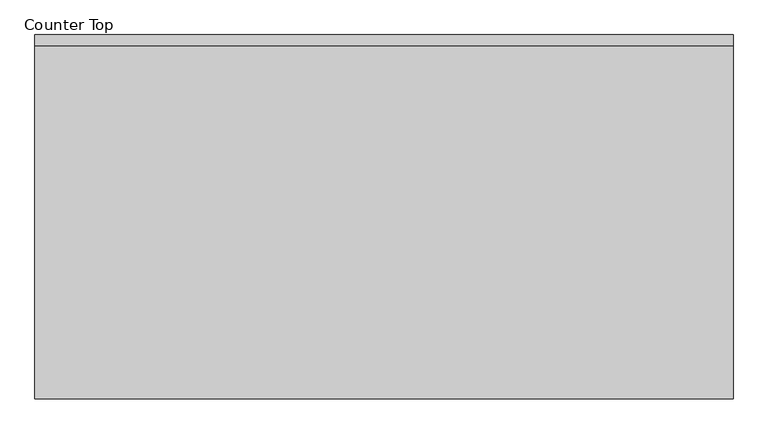
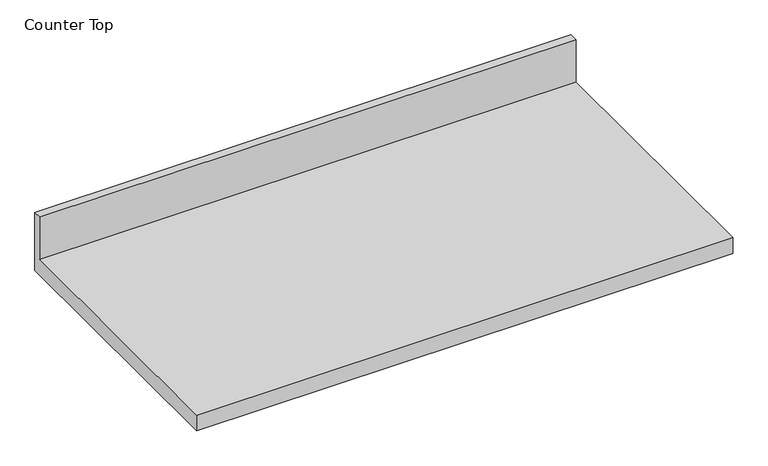
"""IFC4 building model written with IfcOpenShell, lengths in millimetres: furniture geometry, Counter Top."""

from ifc_helpers import new_model, si_unit, frame, origin, place, context, project, spatial, polyline, outline, extrude, source, transform, mapped, element, save


def counter_top_1adf1e72(model_context):
    return source(origin(), model_context, "Body", "SweptSolid", [
        extrude(outline(polyline([(0.0, 1016.0), (0.0, 876.3), (-635.0, 876.3), (-635.0, 914.4), (-19.05, 914.4), (-19.05, 1016.0), (0.0, 1016.0)])), frame((-1200.4622951, 0.0, 0.0), z_axis=(1.0, 0.0, 0.0), x_axis=(0.0, 1.0, 0.0)), (0.0, 0.0, 1.0), 1217.0072912),
    ])


if __name__ == "__main__":
    model = new_model("IFC4")
    model_context = context("Model", 3, world=origin())
    ifc_project = project(units=[si_unit("LENGTHUNIT", "METRE", prefix="MILLI")], contexts=[model_context])
    site = spatial("IfcSite", under=ifc_project)
    building = spatial("IfcBuilding", under=site)
    placement = place(None, origin())
    counter_top_shape = counter_top_1adf1e72(model_context)
    element("IfcFurniture", 1, ObjectType="Counter Top : 24\" Depth Blue Corian", at=placement, inside=building, context=model_context, shape_type="MappedRepresentation", body=[
        mapped(counter_top_shape, transform((0.0, 0.0, 0.0), x_axis=(1.0, 0.0, 0.0), y_axis=(0.0, 1.0, 0.0), z_axis=(0.0, 0.0, 1.0))),
    ])
    save(model, "model.ifc")

# Revit data of these elements
# Type "Counter Top : 24\" Depth Blue Corian"
#   COBie.Type.CreatedBy = "doug.wood@us.ibm.com"
#   COBie.Type.CreatedOn = "2016-04-14T02:07:23"
#   COBie.Type.Name = "Casework_Counter Top_24\" Depth Blue Corian"
#   COBie.Type.Category = "23-40 35 17 47 11 : Kitchen Casework"
#   COBie.Type.Description = "Counter Top_24\" Depth Blue Corian"
#   COBie.Type.Manufacturer = ""
#   COBie.Type.ModelNumber = ""
#   Assembly Code = "C1030400"
#   COBie.Type.ReplacementCost = 0
#   Counter Thickness = 0' - 1 1/2"
#   Depth = 2' - 1"
#   Height = 3' - 0"
#   Length [instance default] = 8' - 0"
#   COBie.Type = no
#   Counter Top Material = Corian - Dusk
# Element 1 (IfcFurniture, "Counter Top : 24\" Depth Blue Corian")
#   Length = 3' - 11.91367"
#   Materials on its faces: "Corian - Dusk"
# Materials
#   "Corian - Dusk": class "Plastic", colour RGB 75 95 146, transparency 0, Manufacturer = "Corning", Cost = 0
